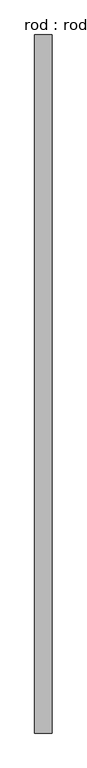
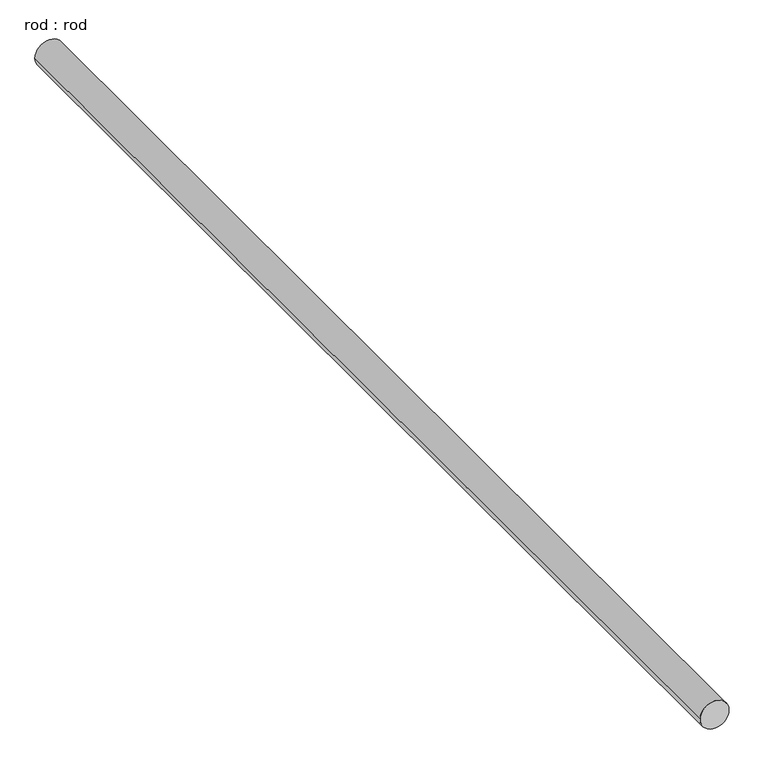
"""IFC4 building model written with IfcOpenShell, lengths in millimetres: proxy geometry, rod : rod."""

from ifc_helpers import new_model, si_unit, point, frame, frame_2d, origin, place, context, project, spatial, circle_curve, trimmed, segment, composite_curve, outline, extrude, source, transform, mapped, element, save


def rod_rod_af5d621a(model_context):
    return source(origin(), model_context, "Body", "SweptSolid", [
        extrude(outline(composite_curve([segment(trimmed(circle_curve(frame_2d((0.0108462, 0.0)), 200.0), [point((0.0108462, 200.0))], [point((0.0108462, -200.0))], False, "CARTESIAN"), True, "CONTINUOUS"), segment(trimmed(circle_curve(frame_2d((0.0108462, 0.0)), 200.0), [point((0.0108462, -200.0))], [point((0.0108462, 200.0))], False, "CARTESIAN"), True, "CONTINUOUS")], self_intersect=False)), frame((0.0, -3880.743025, 0.0), z_axis=(0.0, 1.0, 0.0), x_axis=(0.0, 0.0, 1.0)), (0.0, 0.0, 1.0), 15946.9432808),
    ])


if __name__ == "__main__":
    model = new_model("IFC4")
    model_context = context("Model", 3, world=origin())
    ifc_project = project(units=[si_unit("LENGTHUNIT", "METRE", prefix="MILLI")], contexts=[model_context])
    site = spatial("IfcSite", under=ifc_project)
    building = spatial("IfcBuilding", under=site)
    placement = place(None, origin())
    rod_rod_shape = rod_rod_af5d621a(model_context)
    element("IfcBuildingElementProxy", 1, Name="rod : rod", ObjectType="rod : rod", at=placement, inside=building, context=model_context, shape_type="MappedRepresentation", body=[
        mapped(rod_rod_shape, transform((0.0, 0.0, 0.0), x_axis=(1.0, 0.0, 0.0), y_axis=(0.0, 1.0, 0.0), z_axis=(0.0, 0.0, 1.0))),
    ])
    save(model, "model.ifc")

# Revit data of these elements
# Type "rod : rod"
#   Default Elevation = 0
